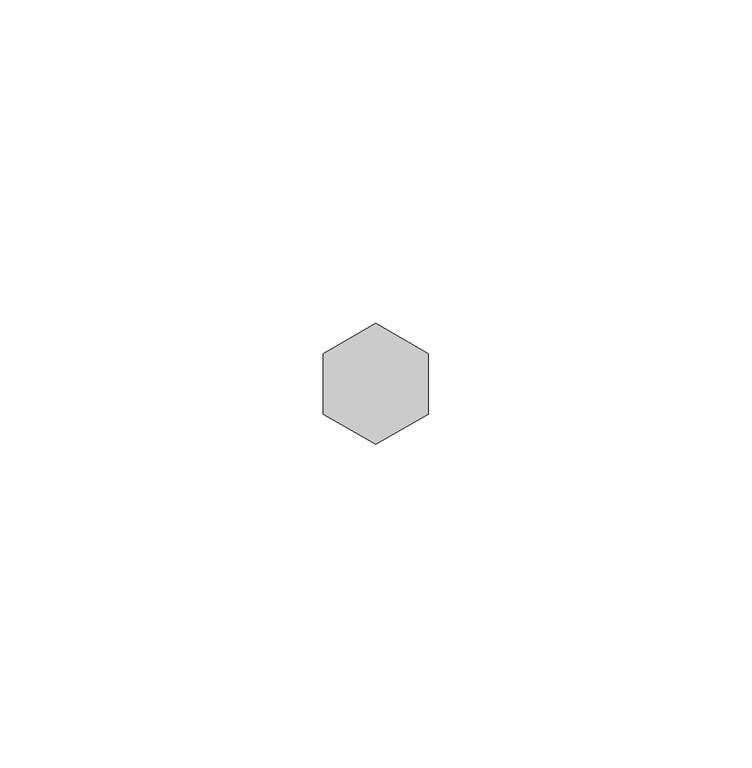
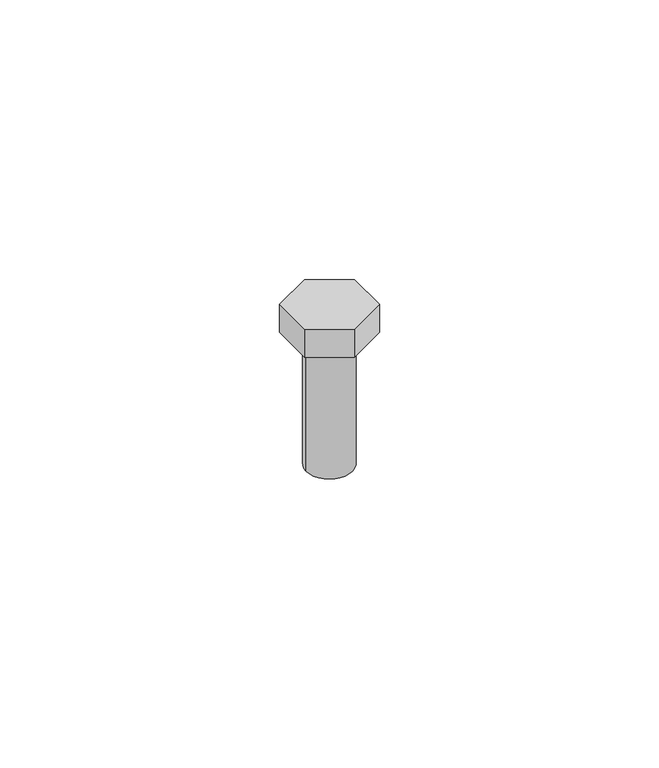
"""IFC4 building model written with IfcOpenShell, lengths in millimetres: proxy geometry, TN_Болт с шестигранной головкой (сборка) : Болт с шестигранной головкой (сборка тип 1)."""

from ifc_helpers import new_model, si_unit, point, frame, origin, origin_with_axes, origin_2d, place, context, project, spatial, polyline, circle_curve, trimmed, segment, composite_curve, outline, extrude, source, transform, mapped, element, save


def generic_models_ea9b8417(model_context):
    return source(origin(), model_context, "Body", "SweptSolid", [
        extrude(outline(polyline([(8.0973375, -4.675), (0.0, -9.35), (-8.0973375, -4.675), (-8.0973375, 4.675), (0.0, 9.35), (8.0973375, 4.675), (8.0973375, -4.675)])), origin_with_axes(), (0.0, 0.0, 1.0), 6.4),
        extrude(outline(composite_curve([segment(trimmed(circle_curve(origin_2d(), 5.0), [point((-5.0, 0.0))], [point((5.0, 0.0))], False, "CARTESIAN"), True, "CONTINUOUS"), segment(trimmed(circle_curve(origin_2d(), 5.0), [point((5.0, 0.0))], [point((-5.0, 0.0))], False, "CARTESIAN"), True, "CONTINUOUS")], self_intersect=False)), frame((0.0, 0.0, -30.0), z_axis=(0.0, 0.0, 1.0), x_axis=(1.0, 0.0, 0.0)), (0.0, 0.0, 1.0), 30.0),
    ])


if __name__ == "__main__":
    model = new_model("IFC4")
    model_context = context("Model", 3, world=origin())
    ifc_project = project(units=[si_unit("LENGTHUNIT", "METRE", prefix="MILLI")], contexts=[model_context])
    site = spatial("IfcSite", under=ifc_project)
    building = spatial("IfcBuilding", under=site)
    placement = place(None, origin())
    generic_models_shape = generic_models_ea9b8417(model_context)
    element("IfcBuildingElementProxy", 1, Name="TN_Болт с шестигранной головкой (сборка) : Болт с шестигранной головкой (сборка тип 1)", ObjectType="TN_Болт с шестигранной головкой (сборка) : Болт с шестигранной головкой (сборка тип 1)", at=placement, inside=building, context=model_context, shape_type="MappedRepresentation", body=[
        mapped(generic_models_shape, transform((0.0, 0.0, 0.0), x_axis=(1.0, 0.0, 0.0), y_axis=(0.0, 1.0, 0.0), z_axis=(0.0, 0.0, 1.0))),
    ])
    save(model, "model.ifc")

# Revit data of these elements
# Type "TN_Болт с шестигранной головкой (сборка) : Болт с шестигранной головкой (сборка тип 1)"
#   Description = "Обеспечивает прочное соединение нескольких деталей, соединение является разъемным. Качество болтового соединения обеспечивается качеством стали, классом прочности и формой болта.\r\nМатериал:\r\nСталь класс прочности 8,8 ГОСТ-7798 (DIN 933).\r\nГальваническое покрытие цинком."
#   Manufacturer = "ТехноНИКОЛЬ"
#   Model = "Комплектующие к опорам"
#   URL = "https://nav.tn.ru/knowledge-base/polimernye-membrany/opory-pod-oborudovanie-na-ploskoy-krovle/?sphrase_id=266812"
#   ADSK_Обозначение = "ТехноНИКОЛЬ"
#   ADSK_Наименование краткое = "M10x30"
#   ADSK_Наименование = "Болт с шестигранной головкой M10x30"
#   ADSK_Масса_Текст = ""
#   ADSK_Марка = "M10x30"
#   ADSK_Код изделия = "660826"
#   ADSK_Завод-изготовитель = "ТехноНИКОЛЬ"
#   ADSK_Единица измерения = "шт."
#   ADSK_Группирование = "Комплектующие к опорам"
#   ADSK_URL страницы изделия = "https://nav.tn.ru/knowledge-base/polimernye-membrany/opory-pod-oborudovanie-na-ploskoy-krovle/?sphrase_id=266812"
#   ADSK_URL документации изделия = ""
#   ADSK_Количество = 1
#   Гайка шестигранная DIN 934 M10 - 8 = no
#   Гайка быстрого монтажа потайная 41 8F M10 = yes
#   ADSK_Материал = TN_СтальГальванизированная_Серый
#   Default Elevation = 0
# Element 1 (IfcBuildingElementProxy, "TN_Болт с шестигранной головкой (сборка) : Болт с шестигранной головкой (сборка тип 1)")
#   Materials on its faces: "TN_СтальГальванизированная_Серый"
# Materials
#   "TN_СтальГальванизированная_Серый": class "Типовые", colour RGB 206 210 213, transparency 0, Cost = 0
